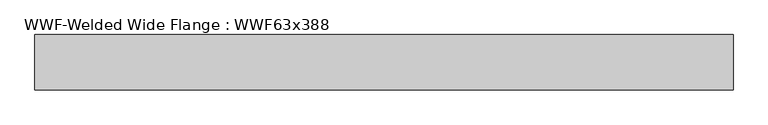
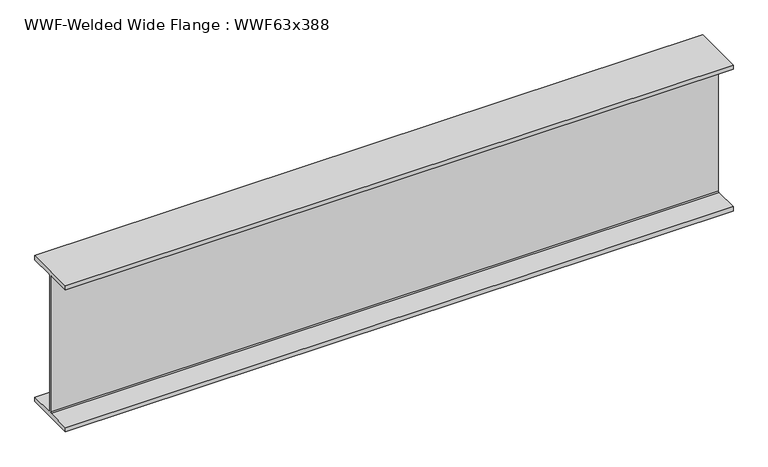
"""IFC4 building model written with IfcOpenShell, lengths in millimetres: beam geometry, WWF-Welded Wide Flange : WWF63x388."""

from ifc_helpers import new_model, si_unit, frame, origin, place, context, project, spatial, polyline, outline, extrude, source, transform, mapped, element, save


def wwf_welded_wide_flange_wwf63x388_99d12122(model_context):
    return source(origin(), model_context, "Body", "SweptSolid", [
        extrude(outline(polyline([(274.955, -755.015), (274.955, -799.973), (-274.955, -799.973), (-274.955, -755.015), (-19.05, -755.015), (-8.001, -743.966), (-8.001, 743.966), (-19.05, 755.015), (-274.955, 755.015), (-274.955, 799.973), (274.955, 799.973), (274.955, 755.015), (19.05, 755.015), (8.001, 743.966), (8.001, -743.966), (19.05, -755.015), (274.955, -755.015)])), frame((-3747.1838372, 0.0, 0.0), z_axis=(1.0, 0.0, 0.0), x_axis=(0.0, 1.0, 0.0)), (0.0, 0.0, 1.0), 6931.7444444),
    ])


if __name__ == "__main__":
    model = new_model("IFC4")
    model_context = context("Model", 3, world=origin())
    ifc_project = project(units=[si_unit("LENGTHUNIT", "METRE", prefix="MILLI")], contexts=[model_context])
    site = spatial("IfcSite", under=ifc_project)
    building = spatial("IfcBuilding", under=site)
    placement = place(None, origin())
    wwf_welded_wide_flange_wwf63x388_shape = wwf_welded_wide_flange_wwf63x388_99d12122(model_context)
    element("IfcBeam", 1, ObjectType="WWF-Welded Wide Flange : WWF63x388", at=placement, inside=building, context=model_context, shape_type="MappedRepresentation", body=[
        mapped(wwf_welded_wide_flange_wwf63x388_shape, transform((0.0, 0.0, 0.0), x_axis=(1.0, 0.0, 0.0), y_axis=(0.0, 1.0, 0.0), z_axis=(0.0, 0.0, 1.0))),
    ])
    save(model, "model.ifc")

# Revit data of these elements
# Type "WWF-Welded Wide Flange : WWF63x388"
#   Assembly Code = "B10"
#   Nominal d = "12"
#   W = 388
#   Length [instance default] = 1524 mm
#   bf = 549.91 mm
#   d = 1599.946 mm
#   k = 19.05 mm
#   tf = 44.958 mm
#   tw = 16.002 mm
#   A = 0.0735482 m²
#   Structural Material [instance default] = Steel ASTM A572
# Element 1 (IfcBeam, "WWF-Welded Wide Flange : WWF63x388")
#   Structural Material = Metal - Steel 43-275
#   Materials on its faces: "Metal - Steel 43-275"
# Materials
#   "Steel ASTM A572": class "Metal", colour RGB 247 247 247, transparency 0, Description = "Structural steel, high strength low alloy, ASTM - A572 - 50", Cost = 0
#   "Metal - Steel 43-275": class "Metal", colour RGB 247 247 247, transparency 0, Cost = 0
